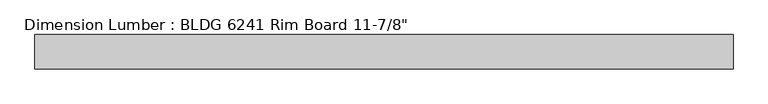
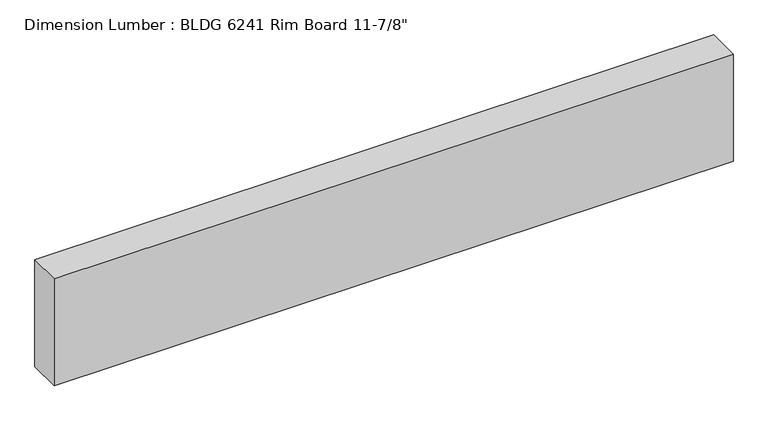
"""IFC4 building model written with IfcOpenShell, lengths in millimetres: beam geometry."""

from ifc_helpers import new_model, si_unit, frame, origin, place, context, project, spatial, polyline, outline, extrude, source, transform, mapped, element, save


def beam_6192414b(model_context):
    return source(origin(), model_context, "Body", "SweptSolid", [
        extrude(outline(polyline([(903.8789755, 44.45), (903.8789755, -44.45), (-906.5092316, -44.45), (-906.5092316, 44.45), (903.8789755, 44.45)])), frame((0.0, 0.0, -150.8125), z_axis=(0.0, 0.0, 1.0), x_axis=(1.0, 0.0, 0.0)), (0.0, 0.0, 1.0), 301.625),
    ])


if __name__ == "__main__":
    model = new_model("IFC4")
    model_context = context("Model", 3, world=origin())
    ifc_project = project(units=[si_unit("LENGTHUNIT", "METRE", prefix="MILLI")], contexts=[model_context])
    site = spatial("IfcSite", under=ifc_project)
    building = spatial("IfcBuilding", under=site)
    placement = place(None, origin())
    beam_shape = beam_6192414b(model_context)
    element("IfcBeam", 1, ObjectType="Dimension Lumber : BLDG 6241 Rim Board 11-7/8\"", at=placement, inside=building, context=model_context, shape_type="MappedRepresentation", body=[
        mapped(beam_shape, transform((0.0, 0.0, 0.0), x_axis=(1.0, 0.0, 0.0), y_axis=(0.0, 1.0, 0.0), z_axis=(0.0, 0.0, 1.0))),
    ])
    save(model, "model.ifc")

# Revit data of these elements
# Type "Dimension Lumber : BLDG 6241 Rim Board 11-7/8\""
#   Assembly Code = "B10"
#   A = 0.273472 SF
#   Length [instance default] = 5' - 0"
#   b = 0' - 3 1/2"
#   d = 0' - 11 7/8"
#   Structural Material [instance default] = Softwood, Lumber
# Element 1 (IfcBeam, "Dimension Lumber : BLDG 6241 Rim Board 11-7/8\"")
#   Materials on its faces: "Softwood, Lumber"
# Materials
#   "Softwood, Lumber": class "Wood", colour RGB 223 192 134, transparency 0, Description = "Pinus Echinata", Cost = 0
